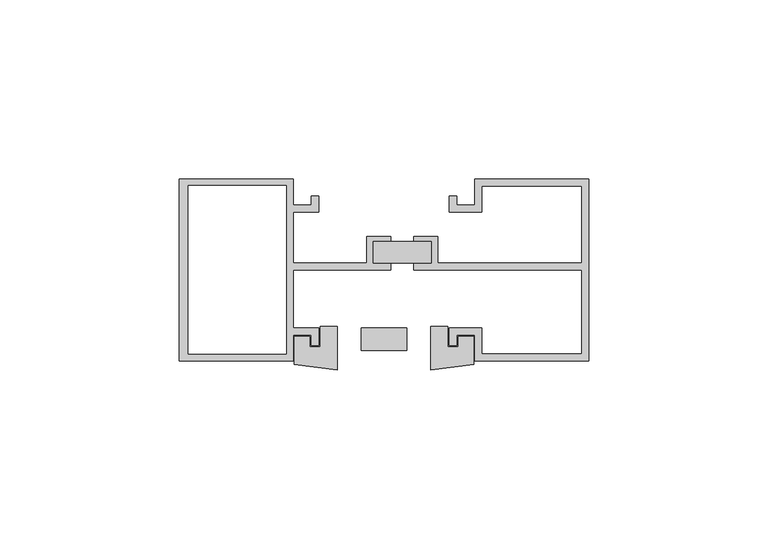
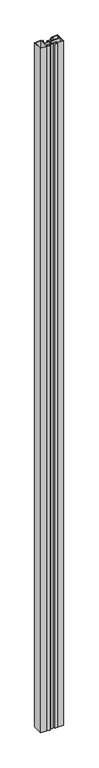
"""IFC4 building model written with IfcOpenShell, lengths in millimetres: proxy geometry, Generic Models 3:Generic Models 1:5:Generic Models 1:5 : Generic Models 3:Generic Models 1:300625:345888:Generic Models 1:5:Generic Models 1:5 : Generic Models 3:Generic Models 1:300625:345888 : Generic Models 3:Generic Models 1:5:Generic Models 1:5 : Generic Models 3:Generic Models 1:300625:345888:7 : Generic Models 3:Generic Models 1:5:Generic Models 1:5 : Generic Models 3:Generic Models 1:300625:345888:Generic Models 1:5:Generic Models 1:5 : Generic Models 3:Generic Models 1:300625:345888 : Generic Models 3:Generic Models 1:5:Generic Models 1:5 : Generic Models 3:Generic Models 1:300625:345888:301574."""

from ifc_helpers import new_model, si_unit, frame, origin, place, context, project, spatial, polyline, outline, extrude, source, transform, mapped, element, save


def generic_models_14010429(model_context):
    return source(origin(), model_context, "Body", "SweptSolid", [
        extrude(outline(polyline([(560302.3728277, -572620.2333389), (560302.3728277, -572614.1535516), (560318.4842638, -572614.1535516), (560318.4842638, -572620.2333389), (560302.3728277, -572620.2333389)])), frame((0.0, 0.0, 66.3122056), z_axis=(0.0, 0.0, 1.0), x_axis=(1.0, 0.0, 0.0)), (0.0, 0.0, 1.0), 3584.971571),
        extrude(outline(polyline([(560298.9867239, -572644.6642543), (560298.9867239, -572638.3207059), (560311.6867239, -572638.3207059), (560311.6867239, -572644.6642543), (560298.9867239, -572644.6642543)])), frame((0.0, 0.0, 66.3122056), z_axis=(0.0, 0.0, 1.0), x_axis=(1.0, 0.0, 0.0)), (0.0, 0.0, 1.0), 3584.971571),
        extrude(outline(polyline([(560287.4942372, -572643.6373715), (560287.4942372, -572637.9238309), (560292.2482931, -572637.9238309), (560292.2482931, -572649.994088), (560280.3504872, -572648.5332212), (560280.3504872, -572640.6935117), (560284.648559, -572640.6935117), (560284.648559, -572643.6373715), (560287.4942372, -572643.6373715)])), frame((0.0, 0.0, 66.3122056), z_axis=(0.0, 0.0, 1.0), x_axis=(1.0, 0.0, 0.0)), (0.0, 0.0, 1.0), 3584.971571),
        extrude(outline(polyline([(560330.3229606, -572648.5332212), (560318.4251548, -572649.994088), (560318.4251548, -572637.9238309), (560323.1792106, -572637.9238309), (560323.1792106, -572643.6373715), (560326.0248888, -572643.6373715), (560326.0248888, -572640.6935117), (560330.3229606, -572640.6935117), (560330.3229606, -572648.5332212)])), frame((0.0, 0.0, 66.3122056), z_axis=(0.0, 0.0, 1.0), x_axis=(1.0, 0.0, 0.0)), (0.0, 0.0, 1.0), 3584.9377944),
        extrude(outline(polyline([(560248.1867239, -572596.7501607), (560279.9536122, -572596.7501607), (560279.9536122, -572603.969908), (560285.045434, -572603.969908), (560285.045434, -572601.4506766), (560287.0973622, -572601.4506766), (560287.0973622, -572606.0218362), (560279.9536122, -572606.0218362), (560279.9536122, -572620.2333389), (560300.4728941, -572620.2333389), (560300.4728941, -572612.8615969), (560307.2366574, -572612.8615969), (560307.2366574, -572614.1535516), (560302.3728277, -572614.1535516), (560302.3728277, -572620.2333389), (560307.2366574, -572620.2333389), (560307.2366574, -572622.1332724), (560279.9536122, -572622.1332724), (560279.9536122, -572638.3207059), (560287.0973622, -572638.3207059), (560287.0973622, -572643.2404965), (560285.045434, -572643.2404965), (560285.045434, -572640.2966367), (560279.9536122, -572640.2966367), (560279.9536122, -572647.5163841), (560248.1867239, -572647.5163841), (560248.1867239, -572596.7501607)]), holes=[polyline([(560278.0536787, -572645.6164506), (560278.0536787, -572598.6500942), (560250.6946362, -572598.6500942), (560250.6946362, -572645.6164506), (560278.0536787, -572645.6164506)])]), frame((0.0, 0.0, 66.3122056), z_axis=(0.0, 0.0, 1.0), x_axis=(1.0, 0.0, 0.0)), (0.0, 0.0, 1.0), 3584.971571),
        extrude(outline(polyline([(560325.6280138, -572643.2404965), (560323.5760856, -572643.2404965), (560323.5760856, -572638.3207059), (560332.6197691, -572638.3207059), (560332.6197691, -572645.606585), (560360.5107931, -572645.606585), (560360.5107931, -572622.1332724), (560313.620434, -572622.1332724), (560313.620434, -572620.2333389), (560318.4842638, -572620.2333389), (560318.4842638, -572614.1535516), (560313.620434, -572614.1535516), (560313.620434, -572612.8615969), (560320.3841973, -572612.8615969), (560320.3841973, -572620.2333389), (560360.5107931, -572620.2333389), (560360.5107931, -572598.6723733), (560332.6197691, -572598.6723733), (560332.6197691, -572606.0218362), (560323.5760856, -572606.0218362), (560323.5760856, -572601.4506766), (560325.6280138, -572601.4506766), (560325.6280138, -572603.969908), (560330.7198356, -572603.969908), (560330.7198356, -572596.7501607), (560362.4867239, -572596.7501607), (560362.4867239, -572647.5163841), (560330.7198356, -572647.5163841), (560330.7198356, -572640.2966367), (560325.6280138, -572640.2966367), (560325.6280138, -572643.2404965)])), frame((0.0, 0.0, 66.3122056), z_axis=(0.0, 0.0, 1.0), x_axis=(1.0, 0.0, 0.0)), (0.0, 0.0, 1.0), 3584.971571),
    ])


if __name__ == "__main__":
    model = new_model("IFC4")
    model_context = context("Model", 3, world=origin())
    ifc_project = project(units=[si_unit("LENGTHUNIT", "METRE", prefix="MILLI")], contexts=[model_context])
    site = spatial("IfcSite", under=ifc_project)
    building = spatial("IfcBuilding", under=site)
    placement = place(None, origin())
    generic_models_shape = generic_models_14010429(model_context)
    element("IfcBuildingElementProxy", 1, Name="Generic Models 3:Generic Models 1:5:Generic Models 1:5 : Generic Models 3:Generic Models 1:300625:345888:Generic Models 1:5:Generic Models 1:5 : Generic Models 3:Generic Models 1:300625:345888 : Generic Models 3:Generic Models 1:5:Generic Models 1:5 : Generic Models 3:Generic Models 1:300625:345888:7 : Generic Models 3:Generic Models 1:5:Generic Models 1:5 : Generic Models 3:Generic Models 1:300625:345888:Generic Models 1:5:Generic Models 1:5 : Generic Models 3:Generic Models 1:300625:345888 : Generic Models 3:Generic Models 1:5:Generic Models 1:5 : Generic Models 3:Generic Models 1:300625:345888:301574", ObjectType="Generic Models 3:Generic Models 1:5:Generic Models 1:5 : Generic Models 3:Generic Models 1:300625:345888:Generic Models 1:5:Generic Models 1:5 : Generic Models 3:Generic Models 1:300625:345888 : Generic Models 3:Generic Models 1:5:Generic Models 1:5 : Generic Models 3:Generic Models 1:300625:345888:7 : Generic Models 3:Generic Models 1:5:Generic Models 1:5 : Generic Models 3:Generic Models 1:300625:345888:Generic Models 1:5:Generic Models 1:5 : Generic Models 3:Generic Models 1:300625:345888 : Generic Models 3:Generic Models 1:5:Generic Models 1:5 : Generic Models 3:Generic Models 1:300625:345888:301574", at=placement, inside=building, context=model_context, shape_type="MappedRepresentation", body=[
        mapped(generic_models_shape, transform((0.0, 0.0, 0.0), x_axis=(1.0, 0.0, 0.0), y_axis=(0.0, 1.0, 0.0), z_axis=(0.0, 0.0, 1.0))),
    ])
    save(model, "model.ifc")

# Revit data of these elements
# Type "Generic Models 3:Generic Models 1:5:Generic Models 1:5 : Generic Models 3:Generic Models 1:300625:345888:Generic Models 1:5:Generic Models 1:5 : Generic Models 3:Generic Models 1:300625:345888 : Generic Models 3:Generic Models 1:5:Generic Models 1:5 : Generic Models 3:Generic Models 1:300625:345888:7 : Generic Models 3:Generic Models 1:5:Generic Models 1:5 : Generic Models 3:Generic Models 1:300625:345888:Generic Models 1:5:Generic Models 1:5 : Generic Models 3:Generic Models 1:300625:345888 : Generic Models 3:Generic Models 1:5:Generic Models 1:5 : Generic Models 3:Generic Models 1:300625:345888:301574"
#   NameOverride = "Generic Models 3:Generic Models 1:5:Generic Models 1:5 : Generic Models 3:Generic Models 1:300625:345888:Generic Models 1:5:Generic Models 1:5 : Generic Models 3:Generic Models 1:300625:345888 : Generic Models 3:Generic Models 1:5:Generic Models 1:5 : Generic Models 3:Generic Models 1:300625:345888:301574"
#   ObjectTypeOverride = "Generic Models 1:5:Generic Models 1:5 : Generic Models 3:Generic Models 1:300625:345888 : Generic Models 3:Generic Models 1:5:Generic Models 1:5 : Generic Models 3:Generic Models 1:300625:345888"
#   Reference = "Generic Models 1"
#   Tag = "301574"
# Element 1 (IfcBuildingElementProxy, "Generic Models 3:Generic Models 1:5:Generic Models 1:5 : Generic Models 3:Generic Models 1:300625:345888:Generic Models 1:5:Generic Models 1:5 : Generic Models 3:Generic Models 1:300625:345888 : Generic Models 3:Generic Models 1:5:Generic Models 1:5 : Generic Models 3:Generic Models 1:300625:345888:7 : Generic Models 3:Generic Models 1:5:Generic Models 1:5 : Generic Models 3:Generic Models 1:300625:345888:Generic Models 1:5:Generic Models 1:5 : Generic Models 3:Generic Models 1:300625:345888 : Generic Models 3:Generic Models 1:5:Generic Models 1:5 : Generic Models 3:Generic Models 1:300625:345888:301574")
#   Materials on its faces: "THERMAL BROKEN ALUMINUM STOREFRONT"
# Materials
#   "THERMAL BROKEN ALUMINUM STOREFRONT": class "Unassigned", colour RGB 244 244 244, transparency 0, Cost = 0
